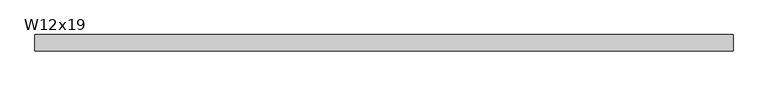
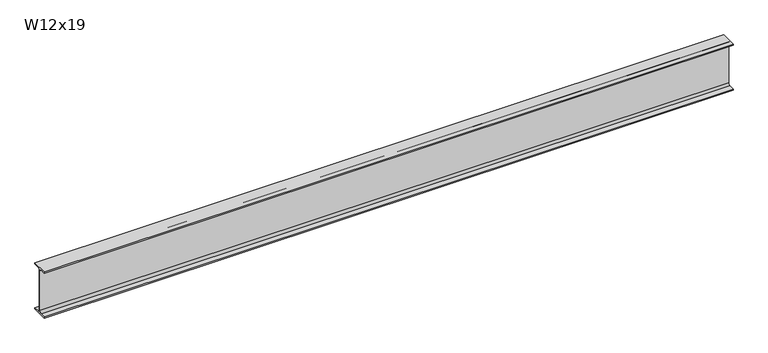
"""IFC4 building model written with IfcOpenShell, lengths in millimetres: beam geometry, RME W-Wide Flange : W12x19."""

import ifcopenshell
import ifcopenshell.guid

model = None  # the IFC model being written
_history = None  # IfcOwnerHistory: only IFC2X3 demands one
_inside = {}  # id of a spatial element -> (the spatial element, [elements in it])
_under = {}  # id of a project, library or spatial element -> (it, [spatial elements below it])
_declared = {}  # id of a project -> (the project, [libraries it declares])
_typed = {}  # id of a type object -> (the type object, [elements of that type])
_made_of = {}  # id of a material, layer set ... -> (it, [elements and type objects made of it])


def new_model(schema):
    """Start an empty IFC model of exactly this schema.

    Asked for "IFC4X3", IfcOpenShell would pick the latest addendum, in which some entities
    have other attributes; the version numbers below select the first issue.
    IFC2X3 requires an IfcOwnerHistory on every rooted entity: one is made here for all.
    """
    global model, _history
    if schema == "IFC4X3":
        model = ifcopenshell.file(schema_version=(4, 3, 0, 0))
    else:
        model = ifcopenshell.file(schema=schema)
    _inside.clear()
    _under.clear()
    _declared.clear()
    _typed.clear()
    _made_of.clear()
    _history = None
    if model.schema == "IFC2X3":
        org = make("IfcOrganization", Name="unknown")
        user = make(
            "IfcPersonAndOrganization",
            ThePerson=make("IfcPerson", FamilyName="unknown"),
            TheOrganization=org,
        )
        app = make(
            "IfcApplication",
            ApplicationDeveloper=org,
            Version="unknown",
            ApplicationFullName="unknown",
            ApplicationIdentifier="unknown",
        )
        _history = make(
            "IfcOwnerHistory",
            OwningUser=user,
            OwningApplication=app,
            ChangeAction="ADDED",
            CreationDate=0,
        )
    return model


def make(cls, **values):
    """One entity of the class cls with the attributes given. An attribute that is None is left unset."""
    return model.create_entity(
        cls, **{name: value for name, value in values.items() if value is not None}
    )


def rooted(cls, **values):
    """An entity with a GlobalId (a new one), such as an element, a storey or a relation."""
    return make(cls, GlobalId=ifcopenshell.guid.new(), OwnerHistory=_history, **values)


def si_unit(unit_type, name, prefix=None):
    """IfcSIUnit, for example si_unit("LENGTHUNIT", "METRE", prefix="MILLI")."""
    return make("IfcSIUnit", UnitType=unit_type, Prefix=prefix, Name=name)


def assignment(units):
    """IfcUnitAssignment: the units of a project."""
    return None if units is None else make("IfcUnitAssignment", Units=units)


def point(xyz):
    """IfcCartesianPoint."""
    return None if xyz is None else make("IfcCartesianPoint", Coordinates=xyz)


def direction(xyz):
    """IfcDirection."""
    return None if xyz is None else make("IfcDirection", DirectionRatios=xyz)


def frame(location, z_axis=None, x_axis=None):
    """IfcAxis2Placement3D, a coordinate frame: its origin and axes. An axis left out is left unset."""
    return make(
        "IfcAxis2Placement3D",
        Location=point(location),
        Axis=direction(z_axis),
        RefDirection=direction(x_axis),
    )


def frame_2d(location, x_axis=None):
    """IfcAxis2Placement2D, a coordinate frame in the plane: its origin and x axis."""
    return make(
        "IfcAxis2Placement2D", Location=point(location), RefDirection=direction(x_axis)
    )


def origin():
    """The frame at (0, 0, 0) with its axes left unset."""
    return frame((0.0, 0.0, 0.0))


def place(relative_to, where):
    """IfcLocalPlacement: puts the frame where relative to a parent placement (None: the world)."""
    return make(
        "IfcLocalPlacement", PlacementRelTo=relative_to, RelativePlacement=where
    )


def context(
    kind, dimensions, precision=None, world=None, true_north=None, identifier=None
):
    """IfcGeometricRepresentationContext, for example the 3D "Model" context."""
    return make(
        "IfcGeometricRepresentationContext",
        ContextIdentifier=identifier,
        ContextType=kind,
        CoordinateSpaceDimension=dimensions,
        Precision=precision,
        WorldCoordinateSystem=world,
        TrueNorth=true_north,
    )


def project(units=None, contexts=None):
    """IfcProject with its units and contexts."""
    return rooted(
        "IfcProject",
        Name="project",
        RepresentationContexts=contexts,
        UnitsInContext=assignment(units),
    )


def spatial(cls, under=None, at=None, **own):
    """A site, building, storey or space (cls), placed at a placement, below another one or the project."""
    s = rooted(cls, ObjectPlacement=at, **own)
    if under is not None:
        _under.setdefault(under.id(), (under, []))[1].append(s)
    return s


def polyline(points):
    """IfcPolyline through the points."""
    return make("IfcPolyline", Points=[point(p) for p in points])


def circle_curve(where, radius):
    """IfcCircle in the frame where."""
    return make("IfcCircle", Position=where, Radius=radius)


def trimmed(basis, trim1, trim2, sense, master):
    """IfcTrimmedCurve: the piece of a basis curve between two trims."""
    return make(
        "IfcTrimmedCurve",
        BasisCurve=basis,
        Trim1=trim1,
        Trim2=trim2,
        SenseAgreement=sense,
        MasterRepresentation=master,
    )


def segment(curve, same_sense, transition):
    """IfcCompositeCurveSegment."""
    return make(
        "IfcCompositeCurveSegment",
        Transition=transition,
        SameSense=same_sense,
        ParentCurve=curve,
    )


def composite_curve(segments, self_intersect=None):
    """IfcCompositeCurve: segments joined end to end."""
    return make("IfcCompositeCurve", Segments=segments, SelfIntersect=self_intersect)


def outline(outer, holes=None, kind="AREA"):
    """IfcArbitraryClosedProfileDef: a profile drawn as a closed curve; with holes, ...WithVoids."""
    if holes is None:
        return make("IfcArbitraryClosedProfileDef", ProfileType=kind, OuterCurve=outer)
    return make(
        "IfcArbitraryProfileDefWithVoids",
        ProfileType=kind,
        OuterCurve=outer,
        InnerCurves=holes,
    )


def extrude(swept, where, along, depth):
    """IfcExtrudedAreaSolid: the profile swept, set in the frame where, extruded along a direction by depth."""
    return make(
        "IfcExtrudedAreaSolid",
        SweptArea=swept,
        Position=where,
        ExtrudedDirection=direction(along),
        Depth=depth,
    )


def shape(context_of_items, identifier, shape_type, items):
    """IfcShapeRepresentation: the items that make up one representation, for example the "Body"."""
    return make(
        "IfcShapeRepresentation",
        ContextOfItems=context_of_items,
        RepresentationIdentifier=identifier,
        RepresentationType=shape_type,
        Items=items,
    )


def source(mapping_origin, context_of_items, identifier, shape_type, items):
    """IfcRepresentationMap: a shape defined once, which mapped items show again and again."""
    return make(
        "IfcRepresentationMap",
        MappingOrigin=mapping_origin,
        MappedRepresentation=shape(context_of_items, identifier, shape_type, items),
    )


def transform(
    local_origin,
    x_axis=None,
    y_axis=None,
    z_axis=None,
    scale=None,
    scale2=None,
    scale3=None,
    uniform=True,
):
    """IfcCartesianTransformationOperator3D, or its non-uniform kind. x_axis, y_axis, z_axis: its Axis1, 2, 3."""
    if uniform:
        return make(
            "IfcCartesianTransformationOperator3D",
            Axis1=direction(x_axis),
            Axis2=direction(y_axis),
            LocalOrigin=point(local_origin),
            Scale=scale,
            Axis3=direction(z_axis),
        )
    return make(
        "IfcCartesianTransformationOperator3DnonUniform",
        Axis1=direction(x_axis),
        Axis2=direction(y_axis),
        LocalOrigin=point(local_origin),
        Scale=scale,
        Axis3=direction(z_axis),
        Scale2=scale2,
        Scale3=scale3,
    )


def mapped(mapping_source, mapping_target):
    """IfcMappedItem: shows the shape of a source again, moved by a transform."""
    return make(
        "IfcMappedItem", MappingSource=mapping_source, MappingTarget=mapping_target
    )


def made_of(thing, what):
    """Note that an element or type object is made of a material, layer set ...; save() writes the relation."""
    if what is not None:
        _made_of.setdefault(what.id(), (what, []))[1].append(thing)
    return thing


def element(
    cls,
    number,
    at=None,
    inside=None,
    cuts=None,
    type_object=None,
    material=None,
    context=None,
    identifier="Body",
    shape_type=None,
    held_by="IfcProductDefinitionShape",
    body=None,
    shapes=None,
    **own,
):
    """One element of the class cls, such as IfcWall. Its Tag is "e" and its number.

    at: its placement. inside: the storey or other place that contains it. cuts: it is an
    opening in that element (IfcRelVoidsElement). A single representation is given by context,
    identifier, shape_type and body (its items); several are given by shapes. held_by: the class
    of the entity that holds the representations. save() writes the other relations.
    """
    e = rooted(cls, Tag="e%d" % number, ObjectPlacement=at, **own)
    if body is not None:
        shapes = [shape(context, identifier, shape_type, body)]
    if shapes is not None:
        e.Representation = make(held_by, Representations=shapes)
    if inside is not None:
        _inside.setdefault(inside.id(), (inside, []))[1].append(e)
    if cuts is not None:
        rooted(
            "IfcRelVoidsElement", RelatingBuildingElement=cuts, RelatedOpeningElement=e
        )
    if type_object is not None:
        _typed.setdefault(type_object.id(), (type_object, []))[1].append(e)
    return made_of(e, material)


def aggregate(whole, parts):
    """IfcRelAggregates: a whole, such as a stair, and the parts it consists of."""
    return rooted("IfcRelAggregates", RelatingObject=whole, RelatedObjects=parts)


def save(model, path):
    """Write the relations noted so far, then the file.

    IfcRelAggregates (storeys below a building ...), IfcRelContainedInSpatialStructure (elements
    in a storey), IfcRelDefinesByType, IfcRelAssociatesMaterial and IfcRelDeclares: one each for
    every whole, place, type object, material and project.
    """
    for whole, parts in _under.values():
        aggregate(whole, parts)
    for where, things in _inside.values():
        rooted(
            "IfcRelContainedInSpatialStructure",
            RelatedElements=things,
            RelatingStructure=where,
        )
    for kind, things in _typed.values():
        rooted("IfcRelDefinesByType", RelatedObjects=things, RelatingType=kind)
    for what, things in _made_of.values():
        rooted("IfcRelAssociatesMaterial", RelatedObjects=things, RelatingMaterial=what)
    for by, libraries in _declared.values():
        rooted("IfcRelDeclares", RelatingContext=by, RelatedDefinitions=libraries)
    model.write(path)


def w12x19_460002c9(model_context):
    return source(origin(), model_context, "Body", "SweptSolid", [
        extrude(outline(composite_curve([segment(polyline([(50.927, -146.05), (50.927, -154.94), (-50.927, -154.94), (-50.927, -146.05), (-16.3195, -146.05)]), True, "CONTINUOUS"), segment(trimmed(circle_curve(frame_2d((-16.3195, -132.715)), 13.335), [point((-16.3195, -146.05))], [point((-2.9845, -132.715))], True, "CARTESIAN"), True, "CONTINUOUS"), segment(polyline([(-2.9845, -132.715), (-2.9845, 132.715)]), True, "CONTINUOUS"), segment(trimmed(circle_curve(frame_2d((-16.3195, 132.715)), 13.335), [point((-2.9845, 132.715))], [point((-16.3195, 146.05))], True, "CARTESIAN"), True, "CONTINUOUS"), segment(polyline([(-16.3195, 146.05), (-50.927, 146.05), (-50.927, 154.94), (50.927, 154.94), (50.927, 146.05), (16.3195, 146.05)]), True, "CONTINUOUS"), segment(trimmed(circle_curve(frame_2d((16.3195, 132.715)), 13.335), [point((16.3195, 146.05))], [point((2.9845, 132.715))], True, "CARTESIAN"), True, "CONTINUOUS"), segment(polyline([(2.9845, 132.715), (2.9845, -132.715)]), True, "CONTINUOUS"), segment(trimmed(circle_curve(frame_2d((16.3195, -132.715)), 13.335), [point((2.9845, -132.715))], [point((16.3195, -146.05))], True, "CARTESIAN"), True, "CONTINUOUS"), segment(polyline([(16.3195, -146.05), (50.927, -146.05)]), True, "CONTINUOUS")], self_intersect=False)), frame((-2206.625, 0.0, 0.0), z_axis=(1.0, 0.0, 0.0), x_axis=(0.0, 1.0, 0.0)), (0.0, 0.0, 1.0), 4359.1706238),
    ])


if __name__ == "__main__":
    model = new_model("IFC4")
    model_context = context("Model", 3, world=origin())
    ifc_project = project(units=[si_unit("LENGTHUNIT", "METRE", prefix="MILLI")], contexts=[model_context])
    site = spatial("IfcSite", under=ifc_project)
    building = spatial("IfcBuilding", under=site)
    placement = place(None, origin())
    w12x19_shape = w12x19_460002c9(model_context)
    element("IfcBeam", 1, ObjectType="RME W-Wide Flange : W12x19", at=placement, inside=building, context=model_context, shape_type="MappedRepresentation", body=[
        mapped(w12x19_shape, transform((0.0, 0.0, 0.0), x_axis=(1.0, 0.0, 0.0), y_axis=(0.0, 1.0, 0.0), z_axis=(0.0, 0.0, 1.0))),
    ])
    save(model, "model.ifc")

# Revit data of these elements
# Type "RME W-Wide Flange : W12x19"
#   WELD P [instance default] = ""
#   WELD LE [instance default] = ""
#   WELD D [instance default] = ""
#   TOP SECTION SIZE [instance default] = ""
#   TOP SECTION LENGTH [instance default] = ""
#   REMARKS [instance default] = ""
#   REINF TYPE [instance default] = ""
#   Nominal Size = "W24"
#   End Bearing Capacity [instance default] = ""
#   BOT SECTION SIZE [instance default] = ""
#   BOT SECTION LENGTH [instance default] = ""
#   Assembly Code = "B10"
#   W = 19
#   Start Extension Calculation [instance default] = 10' - 0"
#   Start Extension [instance default] = -0' - 0 1/2"
#   End Extension Calculation [instance default] = 10' - 0"
#   End Extension [instance default] = -0' - 0 1/2"
#   Length [instance default] = 5' - 0"
#   bf = 0' - 4.01"
#   d = 1' - 0.2"
#   k = 0' - 0 7/8"
#   k2 = 0' - 0.525"
#   tf = 0' - 0.35"
#   tw = 0' - 0.235"
#   A = 0.0386806 SF
#   Structural Material [instance default] = Metal - Steel - ASTM A992
# Element 1 (IfcBeam, "RME W-Wide Flange : W12x19")
#   Length = 14' - 6"
#   Materials on its faces: "Metal - Steel - ASTM A992"
# Materials
#   "Metal - Steel - ASTM A992": class "Metal", colour RGB 255 128 0, transparency 0
